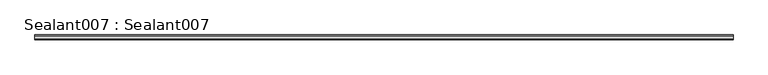
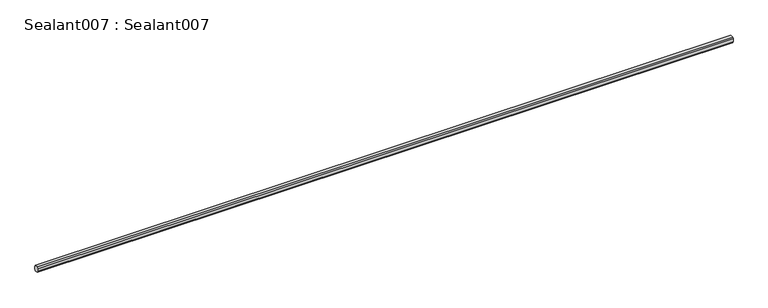
"""IFC4 building model written with IfcOpenShell, lengths in millimetres: proxy geometry, Sealant007 : Sealant007."""

from ifc_helpers import new_model, si_unit, frame, origin, place, context, project, spatial, polyline, outline, extrude, source, transform, mapped, element, save


def sealant007_sealant007_100d3604(model_context):
    return source(origin(), model_context, "Body", "SweptSolid", [
        extrude(outline(polyline([(9516.228715, 37626.0840792), (9518.9316406, 37629.5137666), (9527.4872366, 37629.5137666), (9529.6923147, 37625.4707979), (9529.6923147, 37617.1426729), (9526.9970022, 37612.6075166), (9518.6865234, 37612.6075166), (9516.228715, 37617.1138617), (9516.228715, 37626.0840792)])), frame((-9232.0719278, 0.0, 0.0), z_axis=(1.0, 0.0, 0.0), x_axis=(0.0, 1.0, 0.0)), (0.0, 0.0, 1.0), 1999.85),
    ])


if __name__ == "__main__":
    model = new_model("IFC4")
    model_context = context("Model", 3, world=origin())
    ifc_project = project(units=[si_unit("LENGTHUNIT", "METRE", prefix="MILLI")], contexts=[model_context])
    site = spatial("IfcSite", under=ifc_project)
    building = spatial("IfcBuilding", under=site)
    placement = place(None, origin())
    sealant007_sealant007_shape = sealant007_sealant007_100d3604(model_context)
    element("IfcBuildingElementProxy", 1, Name="Sealant007 : Sealant007", ObjectType="Sealant007 : Sealant007", at=placement, inside=building, context=model_context, shape_type="MappedRepresentation", body=[
        mapped(sealant007_sealant007_shape, transform((0.0, 0.0, 0.0), x_axis=(1.0, 0.0, 0.0), y_axis=(0.0, 1.0, 0.0), z_axis=(0.0, 0.0, 1.0))),
    ])
    save(model, "model.ifc")

# Revit data of these elements
# Type "Sealant007 : Sealant007"
#   NameOverride = "Sealant007"
# Element 1 (IfcBuildingElementProxy, "Sealant007 : Sealant007")
#   Materials on its faces: "BACKER ROD"
# Materials
#   "BACKER ROD": class "Unassigned", colour RGB 214 176 139, transparency 0, Cost = 0
